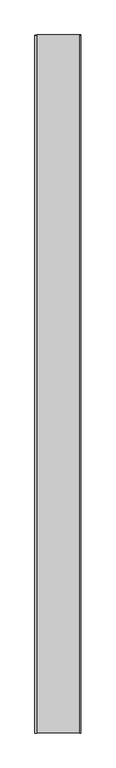
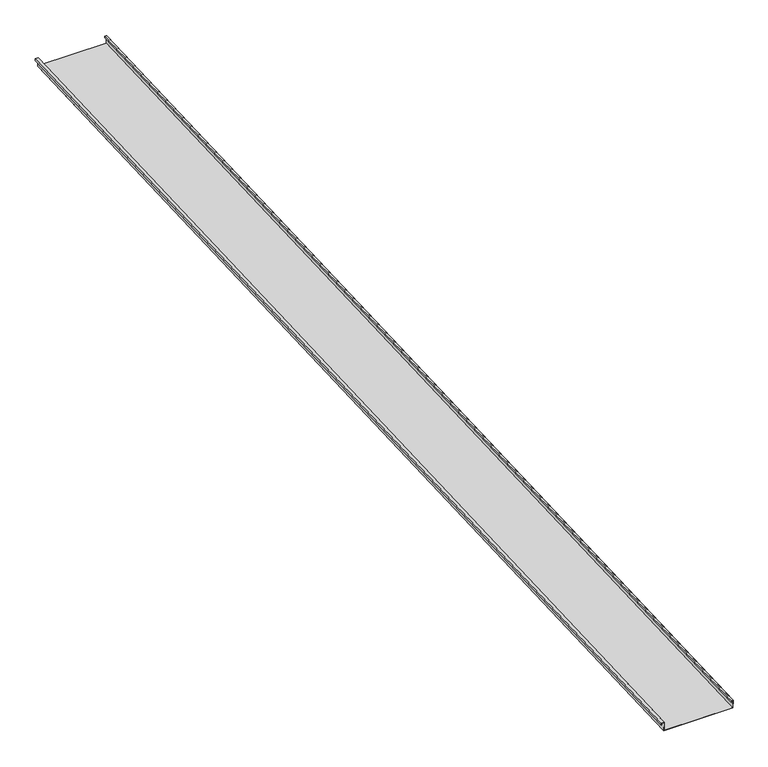
"""IFC4 building model written with IfcOpenShell, lengths in millimetres: proxy geometry, Generic Models 2:Generic Models 2:310765:Generic Models 2:310765 : Generic Models 2:Generic Models 2:310765:133 : Generic Models 2:Generic Models 2:310765:Generic Models 2:310765 : Generic Models 2:Generic Models 2:310765:300385."""

from ifc_helpers import new_model, si_unit, frame, origin, place, context, project, spatial, polyline, outline, extrude, source, transform, mapped, element, save


def generic_models_806f00ea(model_context):
    return source(origin(), model_context, "Body", "SweptSolid", [
        extrude(outline(polyline([(1.5875, 0.0), (1.5875, 50.8), (407.9875, 50.8), (407.9875, 1.5875), (396.875, 1.5875), (396.875, 11.1125), (398.4625, 11.1125), (398.4625, 3.175), (406.4, 3.175), (406.4, 49.2125), (3.175, 49.2125), (3.175, -1.5874999), (-14.2875, -1.5874999), (-14.2875, 9.525), (-12.7, 9.525), (-12.7, 0.0), (1.5875, 0.0)])), frame((659307.3929738, -581354.4345603, 3902.6697972), z_axis=(0.0, 0.9991330730923568, 0.041630544712067834), x_axis=(1.0, 0.0, 0.0)), (0.0, 0.0, 1.0), 6400.8),
    ])


if __name__ == "__main__":
    model = new_model("IFC4")
    model_context = context("Model", 3, world=origin())
    ifc_project = project(units=[si_unit("LENGTHUNIT", "METRE", prefix="MILLI")], contexts=[model_context])
    site = spatial("IfcSite", under=ifc_project)
    building = spatial("IfcBuilding", under=site)
    placement = place(None, origin())
    generic_models_shape = generic_models_806f00ea(model_context)
    element("IfcBuildingElementProxy", 1, Name="Generic Models 2:Generic Models 2:310765:Generic Models 2:310765 : Generic Models 2:Generic Models 2:310765:133 : Generic Models 2:Generic Models 2:310765:Generic Models 2:310765 : Generic Models 2:Generic Models 2:310765:300385", ObjectType="Generic Models 2:Generic Models 2:310765:Generic Models 2:310765 : Generic Models 2:Generic Models 2:310765:133 : Generic Models 2:Generic Models 2:310765:Generic Models 2:310765 : Generic Models 2:Generic Models 2:310765:300385", at=placement, inside=building, context=model_context, shape_type="MappedRepresentation", body=[
        mapped(generic_models_shape, transform((0.0, 0.0, 0.0), x_axis=(1.0, 0.0, 0.0), y_axis=(0.0, 1.0, 0.0), z_axis=(0.0, 0.0, 1.0))),
    ])
    save(model, "model.ifc")

# Revit data of these elements
# Type "Generic Models 2:Generic Models 2:310765:Generic Models 2:310765 : Generic Models 2:Generic Models 2:310765:133 : Generic Models 2:Generic Models 2:310765:Generic Models 2:310765 : Generic Models 2:Generic Models 2:310765:300385"
#   NameOverride = "Generic Models 2:Generic Models 2:310765:Generic Models 2:310765 : Generic Models 2:Generic Models 2:310765:300385"
#   ObjectTypeOverride = "Generic Models 2:310765 : Generic Models 2:Generic Models 2:310765"
#   Reference = "Generic Models 2"
#   Tag = "300385"
# Element 1 (IfcBuildingElementProxy, "Generic Models 2:Generic Models 2:310765:Generic Models 2:310765 : Generic Models 2:Generic Models 2:310765:133 : Generic Models 2:Generic Models 2:310765:Generic Models 2:310765 : Generic Models 2:Generic Models 2:310765:300385")
#   Materials on its faces: "THERMAL BROKEN ALUMINUM STOREFRONT FOR POLYCARBONATE"
# Materials
#   "THERMAL BROKEN ALUMINUM STOREFRONT FOR POLYCARBONATE": class "Unassigned", colour RGB 244 244 244, transparency 0, Keynote = "M07611300.01", Cost = 0
